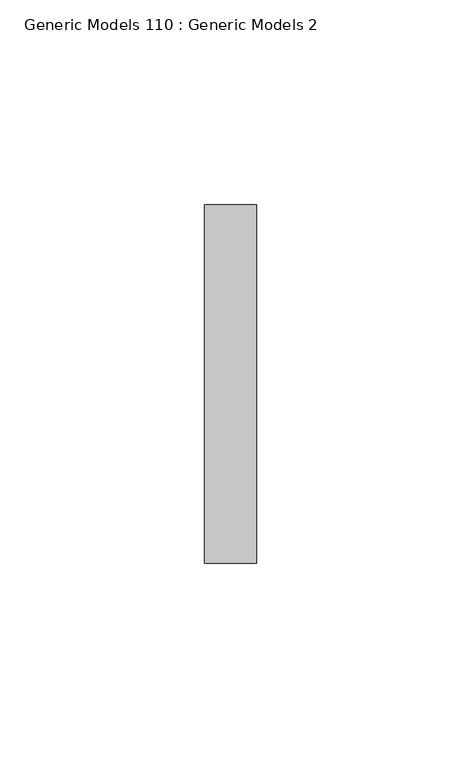
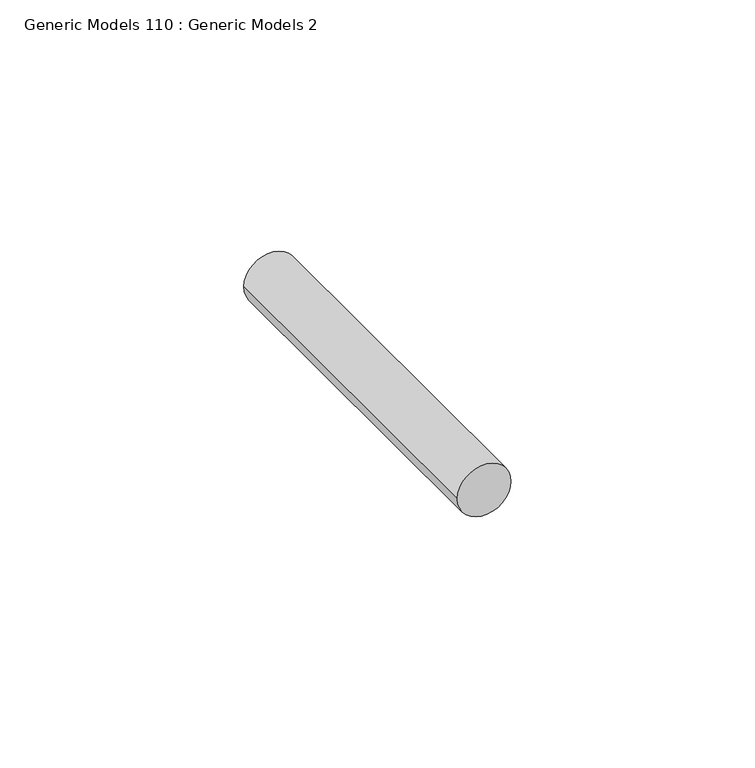
"""IFC4 building model written with IfcOpenShell, lengths in millimetres: proxy geometry, Generic Models 110 : Generic Models 2."""

from ifc_helpers import new_model, si_unit, point, frame, frame_2d, origin, place, context, project, spatial, circle_curve, trimmed, segment, composite_curve, outline, extrude, source, transform, mapped, element, save


def generic_models_110_generic_models_2_2a4c77fe(model_context):
    return source(origin(), model_context, "Body", "SweptSolid", [
        extrude(outline(composite_curve([segment(trimmed(circle_curve(frame_2d((37688.9033735, 6569.3828124)), 6.35), [point((37688.9033735, 6563.0328124))], [point((37688.9033735, 6575.7328124))], False, "CARTESIAN"), True, "CONTINUOUS"), segment(trimmed(circle_curve(frame_2d((37688.9033735, 6569.3828124)), 6.35), [point((37688.9033735, 6575.7328124))], [point((37688.9033735, 6563.0328124))], False, "CARTESIAN"), True, "CONTINUOUS")], self_intersect=False)), frame((0.0, 1848.3666731, 0.0), z_axis=(0.0, 1.0, 0.0), x_axis=(0.0, 0.0, 1.0)), (0.0, 0.0, 1.0), 87.551022),
    ])


if __name__ == "__main__":
    model = new_model("IFC4")
    model_context = context("Model", 3, world=origin())
    ifc_project = project(units=[si_unit("LENGTHUNIT", "METRE", prefix="MILLI")], contexts=[model_context])
    site = spatial("IfcSite", under=ifc_project)
    building = spatial("IfcBuilding", under=site)
    placement = place(None, origin())
    generic_models_110_generic_models_2_shape = generic_models_110_generic_models_2_2a4c77fe(model_context)
    element("IfcBuildingElementProxy", 1, Name="Generic Models 110 : Generic Models 2", ObjectType="Generic Models 110 : Generic Models 2", at=placement, inside=building, context=model_context, shape_type="MappedRepresentation", body=[
        mapped(generic_models_110_generic_models_2_shape, transform((0.0, 0.0, 0.0), x_axis=(1.0, 0.0, 0.0), y_axis=(0.0, 1.0, 0.0), z_axis=(0.0, 0.0, 1.0))),
    ])
    save(model, "model.ifc")

# Revit data of these elements
# Element 1 (IfcBuildingElementProxy, "Generic Models 110 : Generic Models 2")
#   Materials on its faces: "S.S. LAG BOLT - SEE STRUCT. DWGS"
# Materials
#   "S.S. LAG BOLT - SEE STRUCT. DWGS": class "Generic", colour RGB 120 120 120, transparency 0, Cost = 0
